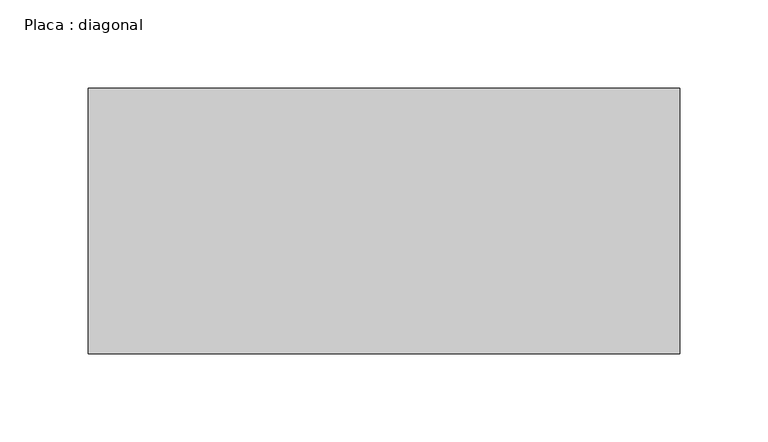
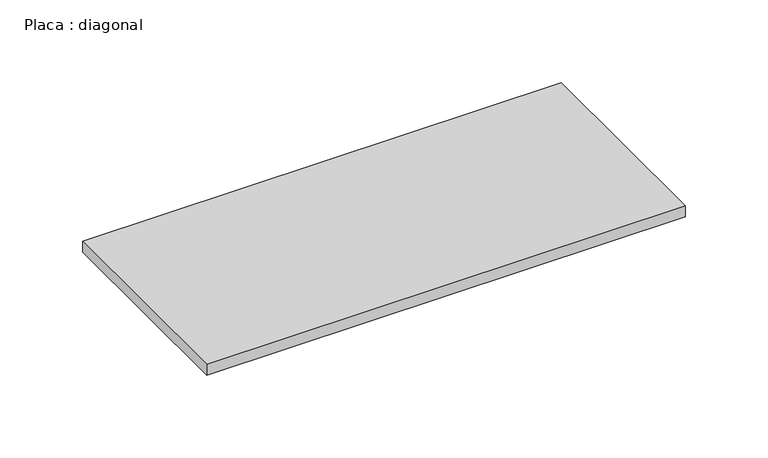
"""IFC4 building model written with IfcOpenShell, lengths in millimetres: beam geometry, Placa : diagonal."""

from ifc_helpers import new_model, si_unit, frame, origin, place, context, project, spatial, polyline, outline, extrude, source, transform, mapped, element, save


def placa_diagonal_ded414cc(model_context):
    return source(origin(), model_context, "Body", "SweptSolid", [
        extrude(outline(polyline([(167.4240165, 75.0), (167.4240165, -75.0), (-167.0675392, -75.0), (-167.0675392, 75.0), (167.4240165, 75.0)])), frame((0.0, 0.0, -4.0), z_axis=(0.0, 0.0, 1.0), x_axis=(1.0, 0.0, 0.0)), (0.0, 0.0, 1.0), 8.0),
    ])


if __name__ == "__main__":
    model = new_model("IFC4")
    model_context = context("Model", 3, world=origin())
    ifc_project = project(units=[si_unit("LENGTHUNIT", "METRE", prefix="MILLI")], contexts=[model_context])
    site = spatial("IfcSite", under=ifc_project)
    building = spatial("IfcBuilding", under=site)
    placement = place(None, origin())
    placa_diagonal_shape = placa_diagonal_ded414cc(model_context)
    element("IfcBeam", 1, ObjectType="Placa : diagonal", at=placement, inside=building, context=model_context, shape_type="MappedRepresentation", body=[
        mapped(placa_diagonal_shape, transform((0.0, 0.0, 0.0), x_axis=(1.0, 0.0, 0.0), y_axis=(0.0, 1.0, 0.0), z_axis=(0.0, 0.0, 1.0))),
    ])
    save(model, "model.ifc")

# Revit data of these elements
# Type "Placa : diagonal"
#   W = 0
#   Length [instance default] = 1.50 m
#   b = 0.15 m
#   d = 0.008 m
#   A = 0 m²
#   Structural Material [instance default] = Aço, 45-345
# Element 1 (IfcBeam, "Placa : diagonal")
#   Materials on its faces: "Aço, 45-345"
# Materials
#   "Aço, 45-345": class "Metal", colour RGB 247 247 247, transparency 0, Description = "Aço 345 MPa", Cost = 0
